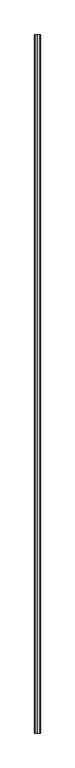
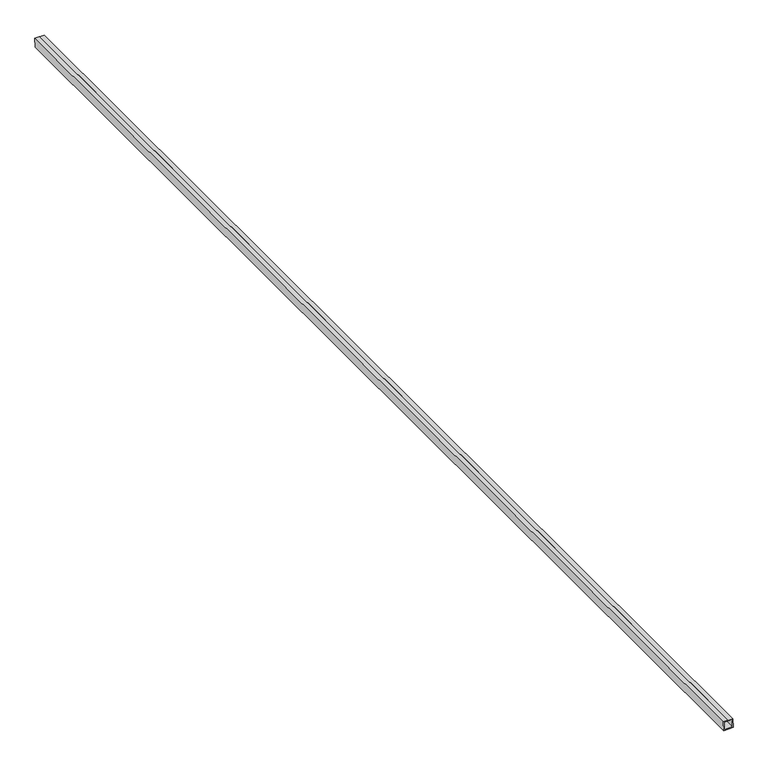
"""IFC4 building model written with IfcOpenShell, lengths in millimetres: proxy geometry, Inner panel:Inner panel:1:Inner panel:1 : Inner panel:Inner panel:300324:2:Inner panel:1:Inner panel:1 : Inner panel:Inner panel:300324:2 : Inner panel:Inner panel:1:Inner panel:1 : Inner panel:Inner panel:300324:300043:35 : Inner panel:Inner panel:1:Inner panel:1 : Inner panel:Inner panel:300324:2:Inner panel:1:Inner panel:1 : Inner panel:Inner panel:300324:2 : Inner panel:Inner panel:1:Inner panel:1 : Inner panel:Inner panel:300324:300043:308120."""

from ifc_helpers import new_model, si_unit, frame, origin, place, context, project, spatial, polyline, outline, extrude, source, transform, mapped, element, save


def generic_models_361145b1(model_context):
    return source(origin(), model_context, "Body", "SweptSolid", [
        extrude(outline(polyline([(3857.794365, 558155.1660493), (3855.4151794, 558155.265182), (3856.0760643, 558171.1264196), (3822.7674654, 558172.5142778), (3821.3796071, 558139.205679), (3854.688206, 558137.8178207), (3855.3490909, 558153.6790583), (3857.7282765, 558153.5799255), (3856.9682589, 558135.3395024), (3818.9012888, 558136.9256261), (3820.4874125, 558174.9925962), (3858.5543826, 558173.4064725), (3857.794365, 558155.1660493)])), frame((0.0, -575657.416384, 0.0), z_axis=(0.0, 1.0, 0.0), x_axis=(0.0, 0.0, 1.0)), (0.0, 0.0, 1.0), 4876.8),
    ])


if __name__ == "__main__":
    model = new_model("IFC4")
    model_context = context("Model", 3, world=origin())
    ifc_project = project(units=[si_unit("LENGTHUNIT", "METRE", prefix="MILLI")], contexts=[model_context])
    site = spatial("IfcSite", under=ifc_project)
    building = spatial("IfcBuilding", under=site)
    placement = place(None, origin())
    generic_models_shape = generic_models_361145b1(model_context)
    element("IfcBuildingElementProxy", 1, Name="Inner panel:Inner panel:1:Inner panel:1 : Inner panel:Inner panel:300324:2:Inner panel:1:Inner panel:1 : Inner panel:Inner panel:300324:2 : Inner panel:Inner panel:1:Inner panel:1 : Inner panel:Inner panel:300324:300043:35 : Inner panel:Inner panel:1:Inner panel:1 : Inner panel:Inner panel:300324:2:Inner panel:1:Inner panel:1 : Inner panel:Inner panel:300324:2 : Inner panel:Inner panel:1:Inner panel:1 : Inner panel:Inner panel:300324:300043:308120", ObjectType="Inner panel:Inner panel:1:Inner panel:1 : Inner panel:Inner panel:300324:2:Inner panel:1:Inner panel:1 : Inner panel:Inner panel:300324:2 : Inner panel:Inner panel:1:Inner panel:1 : Inner panel:Inner panel:300324:300043:35 : Inner panel:Inner panel:1:Inner panel:1 : Inner panel:Inner panel:300324:2:Inner panel:1:Inner panel:1 : Inner panel:Inner panel:300324:2 : Inner panel:Inner panel:1:Inner panel:1 : Inner panel:Inner panel:300324:300043:308120", at=placement, inside=building, context=model_context, shape_type="MappedRepresentation", body=[
        mapped(generic_models_shape, transform((0.0, 0.0, 0.0), x_axis=(1.0, 0.0, 0.0), y_axis=(0.0, 1.0, 0.0), z_axis=(0.0, 0.0, 1.0))),
    ])
    save(model, "model.ifc")

# Revit data of these elements
# Type "Inner panel:Inner panel:1:Inner panel:1 : Inner panel:Inner panel:300324:2:Inner panel:1:Inner panel:1 : Inner panel:Inner panel:300324:2 : Inner panel:Inner panel:1:Inner panel:1 : Inner panel:Inner panel:300324:300043:35 : Inner panel:Inner panel:1:Inner panel:1 : Inner panel:Inner panel:300324:2:Inner panel:1:Inner panel:1 : Inner panel:Inner panel:300324:2 : Inner panel:Inner panel:1:Inner panel:1 : Inner panel:Inner panel:300324:300043:308120"
#   NameOverride = "Inner panel:Inner panel:1:Inner panel:1 : Inner panel:Inner panel:300324:2:Inner panel:1:Inner panel:1 : Inner panel:Inner panel:300324:2 : Inner panel:Inner panel:1:Inner panel:1 : Inner panel:Inner panel:300324:300043:308120"
#   ObjectTypeOverride = "Inner panel:1:Inner panel:1 : Inner panel:Inner panel:300324:2 : Inner panel:Inner panel:1:Inner panel:1 : Inner panel:Inner panel:300324:300043"
#   Reference = "Inner panel"
#   Tag = "308120"
# Element 1 (IfcBuildingElementProxy, "Inner panel:Inner panel:1:Inner panel:1 : Inner panel:Inner panel:300324:2:Inner panel:1:Inner panel:1 : Inner panel:Inner panel:300324:2 : Inner panel:Inner panel:1:Inner panel:1 : Inner panel:Inner panel:300324:300043:35 : Inner panel:Inner panel:1:Inner panel:1 : Inner panel:Inner panel:300324:2:Inner panel:1:Inner panel:1 : Inner panel:Inner panel:300324:2 : Inner panel:Inner panel:1:Inner panel:1 : Inner panel:Inner panel:300324:300043:308120")
#   Materials on its faces: "1 1/2\" X 1 1/2\" x 1/8\" ALUM. TUBE (6061-T6) - (2) #16 WOOD SCREWS WITH 2.5\" EMBED AT EACH GLULAM - (1) SCREW AT ENDS"
# Materials
#   "1 1/2\" X 1 1/2\" x 1/8\" ALUM. TUBE (6061-T6) - (2) #16 WOOD SCREWS WITH 2.5\" EMBED AT EACH GLULAM - (1) SCREW AT ENDS": class "Unassigned", colour RGB 202 201 200, transparency 0, Cost = 0
